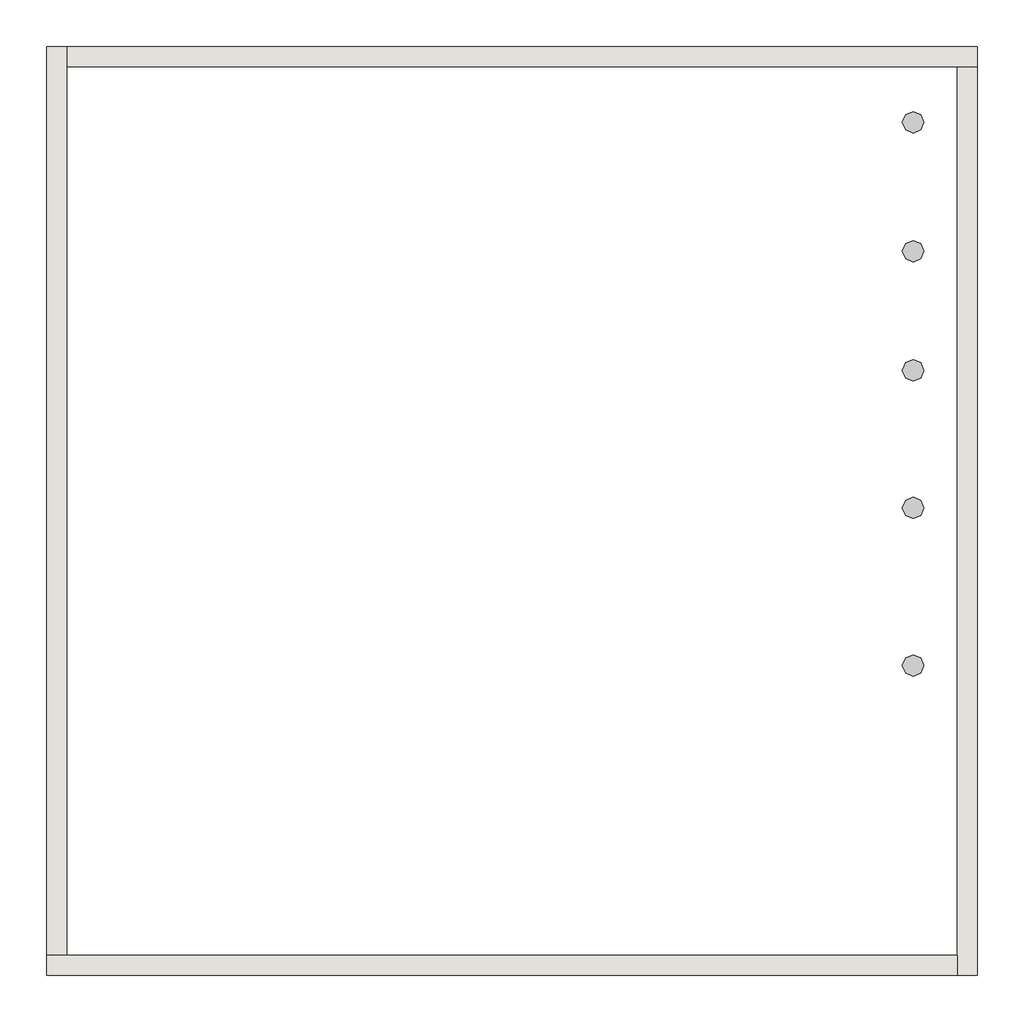
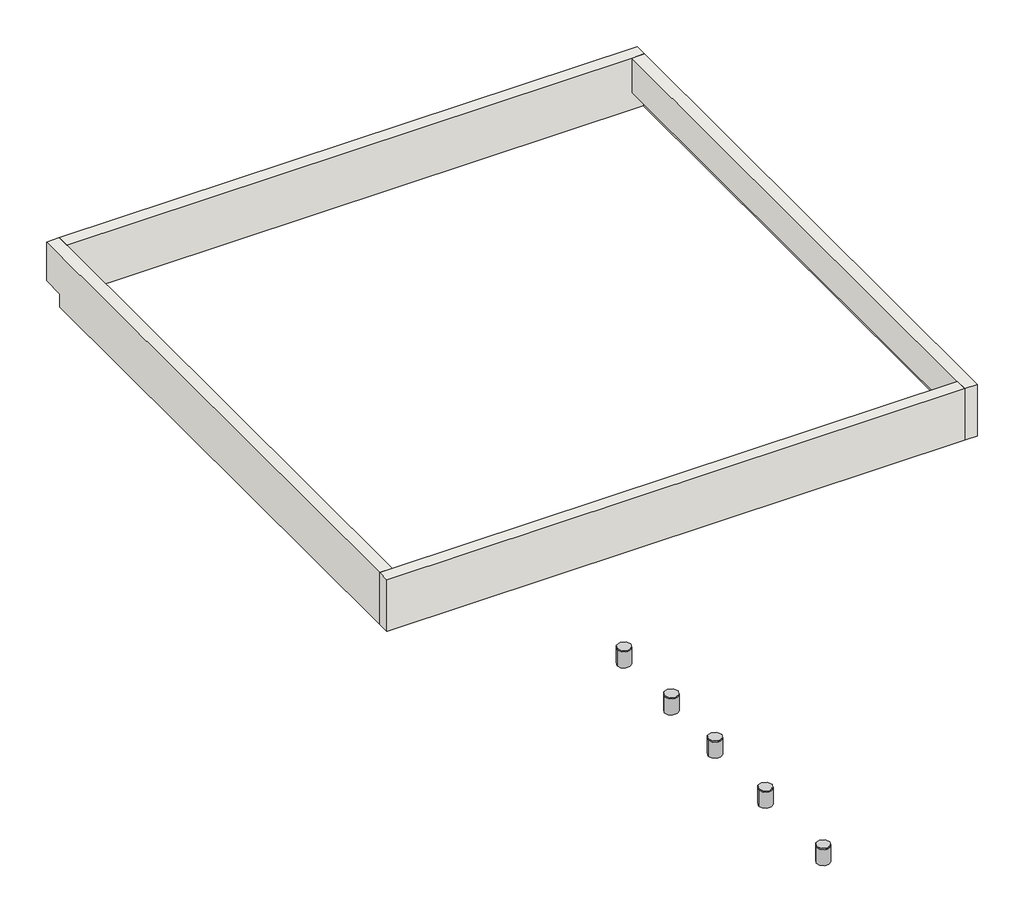
# One storey: 5 light fixtures, 4 walls.
"""IFC4 building model written with IfcOpenShell, lengths in millimetres."""

import ifcopenshell
import ifcopenshell.guid

model = None  # the IFC model being written
_history = None  # IfcOwnerHistory: only IFC2X3 demands one
_inside = {}  # id of a spatial element -> (the spatial element, [elements in it])
_under = {}  # id of a project, library or spatial element -> (it, [spatial elements below it])
_declared = {}  # id of a project -> (the project, [libraries it declares])
_typed = {}  # id of a type object -> (the type object, [elements of that type])
_made_of = {}  # id of a material, layer set ... -> (it, [elements and type objects made of it])


def new_model(schema):
    """Start an empty IFC model of exactly this schema.

    Asked for "IFC4X3", IfcOpenShell would pick the latest addendum, in which some entities
    have other attributes; the version numbers below select the first issue.
    IFC2X3 requires an IfcOwnerHistory on every rooted entity: one is made here for all.
    """
    global model, _history
    if schema == "IFC4X3":
        model = ifcopenshell.file(schema_version=(4, 3, 0, 0))
    else:
        model = ifcopenshell.file(schema=schema)
    _inside.clear()
    _under.clear()
    _declared.clear()
    _typed.clear()
    _made_of.clear()
    _history = None
    if model.schema == "IFC2X3":
        org = make("IfcOrganization", Name="unknown")
        user = make(
            "IfcPersonAndOrganization",
            ThePerson=make("IfcPerson", FamilyName="unknown"),
            TheOrganization=org,
        )
        app = make(
            "IfcApplication",
            ApplicationDeveloper=org,
            Version="unknown",
            ApplicationFullName="unknown",
            ApplicationIdentifier="unknown",
        )
        _history = make(
            "IfcOwnerHistory",
            OwningUser=user,
            OwningApplication=app,
            ChangeAction="ADDED",
            CreationDate=0,
        )
    return model


def make(cls, **values):
    """One entity of the class cls with the attributes given. An attribute that is None is left unset."""
    return model.create_entity(
        cls, **{name: value for name, value in values.items() if value is not None}
    )


def rooted(cls, **values):
    """An entity with a GlobalId (a new one), such as an element, a storey or a relation."""
    return make(cls, GlobalId=ifcopenshell.guid.new(), OwnerHistory=_history, **values)


def si_unit(unit_type, name, prefix=None):
    """IfcSIUnit, for example si_unit("LENGTHUNIT", "METRE", prefix="MILLI")."""
    return make("IfcSIUnit", UnitType=unit_type, Prefix=prefix, Name=name)


def assignment(units):
    """IfcUnitAssignment: the units of a project."""
    return None if units is None else make("IfcUnitAssignment", Units=units)


def point(xyz):
    """IfcCartesianPoint."""
    return None if xyz is None else make("IfcCartesianPoint", Coordinates=xyz)


def direction(xyz):
    """IfcDirection."""
    return None if xyz is None else make("IfcDirection", DirectionRatios=xyz)


def frame(location, z_axis=None, x_axis=None):
    """IfcAxis2Placement3D, a coordinate frame: its origin and axes. An axis left out is left unset."""
    return make(
        "IfcAxis2Placement3D",
        Location=point(location),
        Axis=direction(z_axis),
        RefDirection=direction(x_axis),
    )


def frame_2d(location, x_axis=None):
    """IfcAxis2Placement2D, a coordinate frame in the plane: its origin and x axis."""
    return make(
        "IfcAxis2Placement2D", Location=point(location), RefDirection=direction(x_axis)
    )


def origin():
    """The frame at (0, 0, 0) with its axes left unset."""
    return frame((0.0, 0.0, 0.0))


def origin_2d():
    """The frame at (0, 0) in the plane with its x axis left unset."""
    return frame_2d((0.0, 0.0))


def place(relative_to, where):
    """IfcLocalPlacement: puts the frame where relative to a parent placement (None: the world)."""
    return make(
        "IfcLocalPlacement", PlacementRelTo=relative_to, RelativePlacement=where
    )


def context(
    kind, dimensions, precision=None, world=None, true_north=None, identifier=None
):
    """IfcGeometricRepresentationContext, for example the 3D "Model" context."""
    return make(
        "IfcGeometricRepresentationContext",
        ContextIdentifier=identifier,
        ContextType=kind,
        CoordinateSpaceDimension=dimensions,
        Precision=precision,
        WorldCoordinateSystem=world,
        TrueNorth=true_north,
    )


def project(units=None, contexts=None):
    """IfcProject with its units and contexts."""
    return rooted(
        "IfcProject",
        Name="project",
        RepresentationContexts=contexts,
        UnitsInContext=assignment(units),
    )


def spatial(cls, under=None, at=None, **own):
    """A site, building, storey or space (cls), placed at a placement, below another one or the project."""
    s = rooted(cls, ObjectPlacement=at, **own)
    if under is not None:
        _under.setdefault(under.id(), (under, []))[1].append(s)
    return s


def circle_curve(where, radius):
    """IfcCircle in the frame where."""
    return make("IfcCircle", Position=where, Radius=radius)


def trimmed(basis, trim1, trim2, sense, master):
    """IfcTrimmedCurve: the piece of a basis curve between two trims."""
    return make(
        "IfcTrimmedCurve",
        BasisCurve=basis,
        Trim1=trim1,
        Trim2=trim2,
        SenseAgreement=sense,
        MasterRepresentation=master,
    )


def segment(curve, same_sense, transition):
    """IfcCompositeCurveSegment."""
    return make(
        "IfcCompositeCurveSegment",
        Transition=transition,
        SameSense=same_sense,
        ParentCurve=curve,
    )


def composite_curve(segments, self_intersect=None):
    """IfcCompositeCurve: segments joined end to end."""
    return make("IfcCompositeCurve", Segments=segments, SelfIntersect=self_intersect)


def outline(outer, holes=None, kind="AREA"):
    """IfcArbitraryClosedProfileDef: a profile drawn as a closed curve; with holes, ...WithVoids."""
    if holes is None:
        return make("IfcArbitraryClosedProfileDef", ProfileType=kind, OuterCurve=outer)
    return make(
        "IfcArbitraryProfileDefWithVoids",
        ProfileType=kind,
        OuterCurve=outer,
        InnerCurves=holes,
    )


def extrude(swept, where, along, depth):
    """IfcExtrudedAreaSolid: the profile swept, set in the frame where, extruded along a direction by depth."""
    return make(
        "IfcExtrudedAreaSolid",
        SweptArea=swept,
        Position=where,
        ExtrudedDirection=direction(along),
        Depth=depth,
    )


def faces_of(points, faces, orient=None, outer=None):
    """IfcFace entities. A face is a list of loops; a loop is a list of indices into points, from 0.

    orient and outer hold one flag for each loop. By default every Orientation is true, the
    first loop of a face is its IfcFaceOuterBound and the others are IfcFaceBound.
    """
    made = []
    for i, loops in enumerate(faces):
        bounds = []
        for j, loop in enumerate(loops):
            is_outer = j == 0 if outer is None else outer[i][j]
            bounds.append(
                make(
                    "IfcFaceOuterBound" if is_outer else "IfcFaceBound",
                    Bound=make("IfcPolyLoop", Polygon=[points[k] for k in loop]),
                    Orientation=True if orient is None else orient[i][j],
                )
            )
        made.append(make("IfcFace", Bounds=bounds))
    return made


def faceted_brep(points, faces, orient=None, outer=None, voids=None):
    """IfcFacetedBrep: a solid bounded by flat faces; with voids (closed shells), ...WithVoids."""
    shared = [point(p) for p in points]
    hull = make("IfcClosedShell", CfsFaces=faces_of(shared, faces, orient, outer))
    if voids is None:
        return make("IfcFacetedBrep", Outer=hull)
    return make(
        "IfcFacetedBrepWithVoids",
        Outer=hull,
        Voids=[
            make(cls, CfsFaces=faces_of(shared, fs, o, b)) for cls, fs, o, b in voids
        ],
    )


def shape(context_of_items, identifier, shape_type, items):
    """IfcShapeRepresentation: the items that make up one representation, for example the "Body"."""
    return make(
        "IfcShapeRepresentation",
        ContextOfItems=context_of_items,
        RepresentationIdentifier=identifier,
        RepresentationType=shape_type,
        Items=items,
    )


def source(mapping_origin, context_of_items, identifier, shape_type, items):
    """IfcRepresentationMap: a shape defined once, which mapped items show again and again."""
    return make(
        "IfcRepresentationMap",
        MappingOrigin=mapping_origin,
        MappedRepresentation=shape(context_of_items, identifier, shape_type, items),
    )


def transform(
    local_origin,
    x_axis=None,
    y_axis=None,
    z_axis=None,
    scale=None,
    scale2=None,
    scale3=None,
    uniform=True,
):
    """IfcCartesianTransformationOperator3D, or its non-uniform kind. x_axis, y_axis, z_axis: its Axis1, 2, 3."""
    if uniform:
        return make(
            "IfcCartesianTransformationOperator3D",
            Axis1=direction(x_axis),
            Axis2=direction(y_axis),
            LocalOrigin=point(local_origin),
            Scale=scale,
            Axis3=direction(z_axis),
        )
    return make(
        "IfcCartesianTransformationOperator3DnonUniform",
        Axis1=direction(x_axis),
        Axis2=direction(y_axis),
        LocalOrigin=point(local_origin),
        Scale=scale,
        Axis3=direction(z_axis),
        Scale2=scale2,
        Scale3=scale3,
    )


def mapped(mapping_source, mapping_target):
    """IfcMappedItem: shows the shape of a source again, moved by a transform."""
    return make(
        "IfcMappedItem", MappingSource=mapping_source, MappingTarget=mapping_target
    )


def made_of(thing, what):
    """Note that an element or type object is made of a material, layer set ...; save() writes the relation."""
    if what is not None:
        _made_of.setdefault(what.id(), (what, []))[1].append(thing)
    return thing


def element(
    cls,
    number,
    at=None,
    inside=None,
    cuts=None,
    type_object=None,
    material=None,
    context=None,
    identifier="Body",
    shape_type=None,
    held_by="IfcProductDefinitionShape",
    body=None,
    shapes=None,
    **own,
):
    """One element of the class cls, such as IfcWall. Its Tag is "e" and its number.

    at: its placement. inside: the storey or other place that contains it. cuts: it is an
    opening in that element (IfcRelVoidsElement). A single representation is given by context,
    identifier, shape_type and body (its items); several are given by shapes. held_by: the class
    of the entity that holds the representations. save() writes the other relations.
    """
    e = rooted(cls, Tag="e%d" % number, ObjectPlacement=at, **own)
    if body is not None:
        shapes = [shape(context, identifier, shape_type, body)]
    if shapes is not None:
        e.Representation = make(held_by, Representations=shapes)
    if inside is not None:
        _inside.setdefault(inside.id(), (inside, []))[1].append(e)
    if cuts is not None:
        rooted(
            "IfcRelVoidsElement", RelatingBuildingElement=cuts, RelatedOpeningElement=e
        )
    if type_object is not None:
        _typed.setdefault(type_object.id(), (type_object, []))[1].append(e)
    return made_of(e, material)


def aggregate(whole, parts):
    """IfcRelAggregates: a whole, such as a stair, and the parts it consists of."""
    return rooted("IfcRelAggregates", RelatingObject=whole, RelatedObjects=parts)


def save(model, path):
    """Write the relations noted so far, then the file.

    IfcRelAggregates (storeys below a building ...), IfcRelContainedInSpatialStructure (elements
    in a storey), IfcRelDefinesByType, IfcRelAssociatesMaterial and IfcRelDeclares: one each for
    every whole, place, type object, material and project.
    """
    for whole, parts in _under.values():
        aggregate(whole, parts)
    for where, things in _inside.values():
        rooted(
            "IfcRelContainedInSpatialStructure",
            RelatedElements=things,
            RelatingStructure=where,
        )
    for kind, things in _typed.values():
        rooted("IfcRelDefinesByType", RelatedObjects=things, RelatingType=kind)
    for what, things in _made_of.values():
        rooted("IfcRelAssociatesMaterial", RelatedObjects=things, RelatingMaterial=what)
    for by, libraries in _declared.values():
        rooted("IfcRelDeclares", RelatingContext=by, RelatedDefinitions=libraries)
    model.write(path)


def m_downlight_recessed_can_152mm_incandescent_120v_9e946963(model_context):
    return source(origin(), model_context, "Body", "SweptSolid", [
        extrude(outline(composite_curve([segment(trimmed(circle_curve(origin_2d(), 75.0), [point((-75.0, 0.0))], [point((75.0, 0.0))], False, "CARTESIAN"), True, "CONTINUOUS"), segment(trimmed(circle_curve(origin_2d(), 75.0), [point((75.0, 0.0))], [point((-75.0, 0.0))], False, "CARTESIAN"), True, "CONTINUOUS")], self_intersect=False)), frame((0.0, 0.0, 2625.7), z_axis=(0.0, 0.0, 1.0), x_axis=(1.0, 0.0, 0.0)), (0.0, 0.0, 1.0), 12.7),
        extrude(outline(composite_curve([segment(trimmed(circle_curve(origin_2d(), 75.0), [point((-75.0, 0.0))], [point((75.0, 0.0))], False, "CARTESIAN"), True, "CONTINUOUS"), segment(trimmed(circle_curve(origin_2d(), 75.0), [point((75.0, 0.0))], [point((-75.0, 0.0))], False, "CARTESIAN"), True, "CONTINUOUS")], self_intersect=False), holes=[composite_curve([segment(trimmed(circle_curve(origin_2d(), 62.3), [point((-62.3, 0.0))], [point((62.3, 0.0))], True, "CARTESIAN"), True, "CONTINUOUS"), segment(trimmed(circle_curve(origin_2d(), 62.3), [point((62.3, 0.0))], [point((-62.3, 0.0))], True, "CARTESIAN"), True, "CONTINUOUS")], self_intersect=False)]), frame((0.0, 0.0, 2438.4), z_axis=(0.0, 0.0, 1.0), x_axis=(1.0, 0.0, 0.0)), (0.0, 0.0, 1.0), 187.3),
    ])


model = new_model("IFC4")

# Units and contexts
model_context = context("Model", 3, world=origin())
ifc_project = project(units=[si_unit("LENGTHUNIT", "METRE", prefix="MILLI")], contexts=[model_context])

# Site, building, storey
site = spatial("IfcSite", under=ifc_project)
building = spatial("IfcBuilding", under=site)
storey = spatial("IfcBuildingStorey", under=building, Name="MUMTY TOC", Elevation=9398.0)

# Light fixtures
placement = place(None, origin())
m_downlight_recessed_can_152mm_incandescent_120v_shape = m_downlight_recessed_can_152mm_incandescent_120v_9e946963(model_context)
element("IfcLightFixture", 1, ObjectType="M_Downlight - Recessed Can : 152mm Incandescent - 120V", at=placement, inside=storey, context=model_context, shape_type="MappedRepresentation", body=[
    mapped(m_downlight_recessed_can_152mm_incandescent_120v_shape, transform((16861.6388874, -514.3, 711.6), x_axis=(1.0, 0.0, 0.0), y_axis=(0.0, 1.0, 0.0), z_axis=(0.0, 0.0, 1.0))),
])
element("IfcLightFixture", 2, ObjectType="M_Downlight - Recessed Can : 152mm Incandescent - 120V", at=placement, inside=storey, context=model_context, shape_type="MappedRepresentation", body=[
    mapped(m_downlight_recessed_can_152mm_incandescent_120v_shape, transform((16861.6388874, -1414.3, 711.6), x_axis=(1.0, 0.0, 0.0), y_axis=(0.0, 1.0, 0.0), z_axis=(0.0, 0.0, 1.0))),
])
element("IfcLightFixture", 3, ObjectType="M_Downlight - Recessed Can : 152mm Incandescent - 120V", at=placement, inside=storey, context=model_context, shape_type="MappedRepresentation", body=[
    mapped(m_downlight_recessed_can_152mm_incandescent_120v_shape, transform((16861.6388874, -2245.65, 711.6), x_axis=(1.0, 0.0, 0.0), y_axis=(0.0, 1.0, 0.0), z_axis=(0.0, 0.0, 1.0))),
])
element("IfcLightFixture", 4, ObjectType="M_Downlight - Recessed Can : 152mm Incandescent - 120V", at=placement, inside=storey, context=model_context, shape_type="MappedRepresentation", body=[
    mapped(m_downlight_recessed_can_152mm_incandescent_120v_shape, transform((16861.6388874, -3205.1, 711.6), x_axis=(1.0, 0.0, 0.0), y_axis=(0.0, 1.0, 0.0), z_axis=(0.0, 0.0, 1.0))),
])
element("IfcLightFixture", 5, ObjectType="M_Downlight - Recessed Can : 152mm Incandescent - 120V", at=placement, inside=storey, context=model_context, shape_type="MappedRepresentation", body=[
    mapped(m_downlight_recessed_can_152mm_incandescent_120v_shape, transform((16861.6388874, -4305.1, 711.6), x_axis=(1.0, 0.0, 0.0), y_axis=(0.0, 1.0, 0.0), z_axis=(0.0, 0.0, 1.0))),
])

# Walls
element("IfcWall", 6, ObjectType="PTS- BR- 4.5\"", at=placement, inside=storey, context=model_context, shape_type="Brep", body=[
    faceted_brep([(10818.1, -6466.6, 9248.0), (17170.4, -6466.6, 9248.0), (17170.4, -6466.6, 9848.0), (10818.1, -6466.6, 9848.0), (10818.1, -6326.9, 9248.0), (10818.1, -6326.9, 9848.0), (10957.8, -6326.9, 9848.0), (17170.4, -6326.9, 9848.0), (17170.4, -6326.9, 9248.0), (10833.1, -6326.9, 9248.0)], [[[0, 1, 2, 3]], [[4, 5, 6, 7, 8, 9]], [[1, 0, 4, 9, 8]], [[3, 2, 7, 6, 5]], [[0, 3, 5, 4]], [[2, 1, 8, 7]]]),
])
element("IfcWall", 7, ObjectType="PTS- BR- 4.5\"", at=placement, inside=storey, context=model_context, shape_type="Brep", body=[
    faceted_brep([(10818.1, -241.3, 9248.0), (10818.1, -2563.1, 9248.0), (10818.1, -6326.9, 9248.0), (10818.1, -6326.9, 9848.0), (10818.1, 12.7, 9848.0), (10818.1, 12.7, 9398.0), (10818.1, -241.3, 9398.0), (10957.8, 12.7, 9848.0), (10957.8, -127.0, 9848.0), (10957.8, -6326.9, 9848.0), (10957.8, -6326.9, 9448.8), (10957.8, 12.7, 9448.8), (10833.1, -241.3, 9248.0), (10833.1, -2563.1, 9248.0), (10833.1, -6326.9, 9248.0), (10833.1, -6326.9, 9448.8), (10833.1, 12.7, 9398.0), (10833.1, -241.3, 9398.0), (10833.1, 12.7, 9448.8)], [[[0, 1, 2, 3, 4, 5, 6]], [[7, 8, 9, 10, 11]], [[2, 1, 0, 12, 13, 14]], [[4, 3, 9, 8, 7]], [[3, 2, 14, 15, 10, 9]], [[6, 5, 16, 17]], [[0, 6, 17, 12]], [[5, 4, 7, 11, 18, 16]], [[15, 18, 11, 10]], [[18, 15, 14, 13, 12, 17, 16]]]),
])
element("IfcWall", 8, ObjectType="PTS- BR- 4.5\"", at=placement, inside=storey, context=model_context, shape_type="Brep", body=[
    faceted_brep([(17310.1, 12.7, 9248.0), (10957.8, 12.7, 9248.0), (10957.8, 12.7, 9448.8), (10957.8, 12.7, 9848.0), (17310.1, 12.7, 9848.0), (17310.1, -127.0, 9248.0), (17310.1, -127.0, 9848.0), (17170.4, -127.0, 9848.0), (10957.8, -127.0, 9848.0), (10957.8, -127.0, 9248.0), (17297.4, -127.0, 9248.0)], [[[0, 1, 2, 3, 4]], [[5, 6, 7, 8, 9, 10]], [[1, 0, 5, 10, 9]], [[4, 3, 8, 7, 6]], [[0, 4, 6, 5]], [[1, 9, 8, 3, 2]]]),
])
element("IfcWall", 9, ObjectType="PTS- BR- 4.5\"", at=placement, inside=storey, context=model_context, shape_type="Brep", body=[
    faceted_brep([(17310.1, -6466.6, 9248.0), (17310.1, -127.0, 9248.0), (17310.1, -127.0, 9848.0), (17310.1, -6466.6, 9848.0), (17170.4, -6466.6, 9848.0), (17170.4, -6326.9, 9848.0), (17170.4, -127.0, 9848.0), (17170.4, -127.0, 9448.8), (17170.4, -6451.6, 9448.8), (17170.4, -6451.6, 9248.0), (17170.4, -6466.6, 9248.0), (17297.4, -6451.6, 9248.0), (17297.4, -127.0, 9248.0), (17297.4, -127.0, 9448.8), (17297.4, -6451.6, 9448.8)], [[[0, 1, 2, 3]], [[4, 5, 6, 7, 8, 9, 10]], [[1, 0, 10, 9, 11, 12]], [[3, 2, 6, 5, 4]], [[0, 3, 4, 10]], [[2, 1, 12, 13, 7, 6]], [[13, 14, 8, 7]], [[14, 13, 12, 11]], [[8, 14, 11, 9]]]),
])

save(model, "model.ifc")

# Revit data of these elements
# Type "M_Downlight - Recessed Can : 152mm Incandescent - 120V"
#   Assembly Code = "D5020220"
#   Lamp = "A-19"
#   Wattage = 60 W
#   built-in parameter 1150110 = 1 (stored number, unit not read)
#   built-in parameter 1114217 = 1 (stored number, unit not read)
#   built-in parameter 1150109 = 1 (stored number, unit not read)
#   built-in parameter 1150113 = 1 (stored number, unit not read)
#   Tilt Angle = 90.00°
#   built-in parameter 1010507 = 1.5708 (stored number, unit not read)
#   built-in parameter 1010506 = 0.523599 (stored number, unit not read)
#   Recessing Radius = 75 mm
#   Recessing Inner Radius = 62.3 mm
#   built-in parameter 1150115 = 1 (stored number, unit not read)
#   built-in parameter 1150105 = 2858.75 (stored number, unit not read)
#   Light Source Symbol Length = 3048 mm
#   built-in parameter 1150112 = 1 (stored number, unit not read)
#   built-in parameter 1150114 = 1 (stored number, unit not read)
#   built-in parameter 1150107 = 2800 (stored number, unit not read)
#   built-in parameter 1150106 = 28.5875 (stored number, unit not read)
#   built-in parameter 1150104 = 1.32387 (stored number, unit not read)
#   Ballast Voltage = 120 V
#   built-in parameter 1114218 = 1 (stored number, unit not read)
#   built-in parameter 1150133 = 10 (stored number, unit not read)
#   Recessing Height = 200 mm
#   Recessing Diameter = 150 mm
#   Lumens = 855 lm
#   Apparent Load = 60 VA
#   built-in parameter 1150134 = 4
#   built-in parameter 1150137 = 1
#   Color Filter = 16777215
#   Ballast Number of Poles = 1
#   Material = none
#   Load Classification = Lighting - Dwelling Unit
#   Dimming Lamp Color Temperature Shift = (empty or 0)
#   Default Elevation = 0
#   Wattage Comments = ""
# Type "PTS- BR- 4.5\""
#   Assembly Code = "B2010"
#   Layers, outside or top first: 12.7 mm "PLASTER MAT" (function 4); 114.3 mm "Brick, Common" (function 1); 12.7 mm "PLASTER MAT" (function 4)
# Element 1 (IfcLightFixture, "M_Downlight - Recessed Can : 152mm Incandescent - 120V")
#   Mark = "1"
#   Phase Created = New Construction
# Element 2 (IfcLightFixture, "M_Downlight - Recessed Can : 152mm Incandescent - 120V")
#   Mark = "2"
#   Phase Created = New Construction
# Element 3 (IfcLightFixture, "M_Downlight - Recessed Can : 152mm Incandescent - 120V")
#   Mark = "3"
#   Phase Created = New Construction
# Element 4 (IfcLightFixture, "M_Downlight - Recessed Can : 152mm Incandescent - 120V")
#   Mark = "4"
#   Phase Created = New Construction
# Element 5 (IfcLightFixture, "M_Downlight - Recessed Can : 152mm Incandescent - 120V")
#   Mark = "5"
#   Phase Created = New Construction
# Elements 6, 9 (IfcWall, "PTS- BR- 4.5\"")
#   built-in parameter 1001111 = -150 mm
#   Top Offset = 0 mm
#   Base Offset = -150 mm
#   Unconnected Height = 600 mm
#   wall height = 600 mm
#   Phase Created = New Construction
#   Base Constraint = MUMTY TOC
#   Materials on its faces: "Default Wall", "P6", "PLASTER MAT"
# Elements 7, 8 (IfcWall, "PTS- BR- 4.5\"")
#   built-in parameter 1001111 = -150 mm
#   Top Offset = 0 mm
#   Base Offset = -150 mm
#   Unconnected Height = 600 mm
#   wall height = 600 mm
#   Phase Created = New Construction
#   Base Constraint = MUMTY TOC
#   Materials on its faces: "Default Wall", "PLASTER MAT", "P6"
# Materials
#   "PLASTER MAT": class "Generic", colour RGB 120 120 120, transparency 0, Cost = 0
#   "Brick, Common": class "Masonry", colour RGB 192 192 192, transparency 0, Description = "Common brick", Cost = 0
#   "Default Wall": class "Miscellaneous", colour RGB 128 128 128, transparency 0, Cost = 0
#   "P6": class "Generic", colour RGB 120 120 120, transparency 0, Cost = 0
